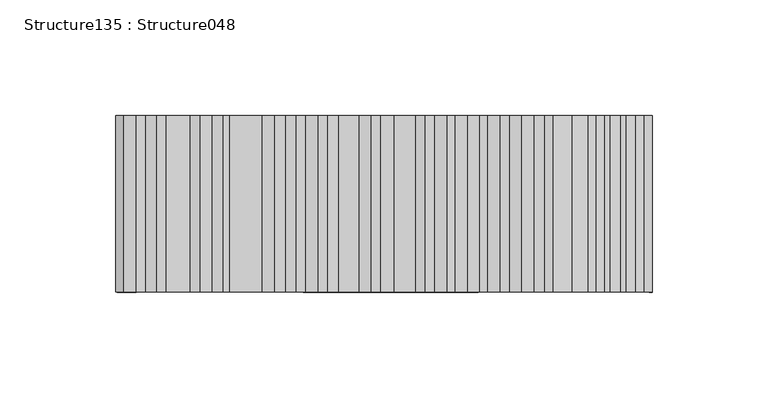
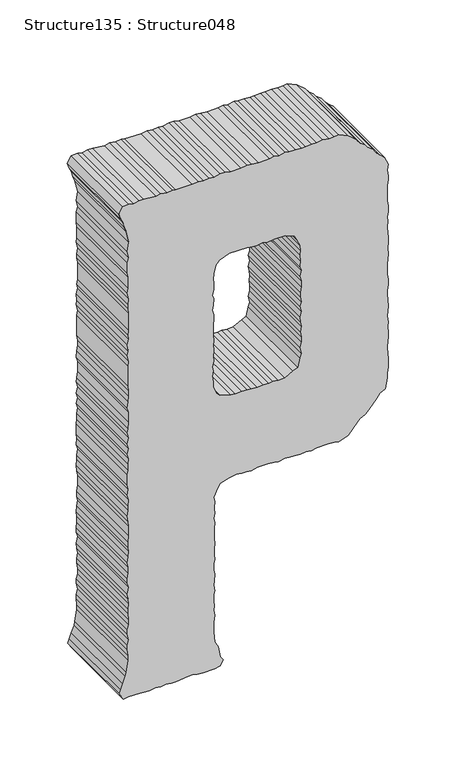
"""IFC4 building model written with IfcOpenShell, lengths in millimetres: proxy geometry, Structure135 : Structure048."""

from ifc_helpers import new_model, si_unit, frame, origin, place, context, project, spatial, polyline, outline, extrude, source, transform, mapped, element, save


def structure135_structure048_a458fe5a(model_context):
    return source(origin(), model_context, "Body", "SweptSolid", [
        extrude(outline(polyline([(3996.390138, -43296.1725089), (3996.390138, -43304.9753692), (3997.5486624, -43309.6560005), (3997.5486624, -43313.755765), (3996.390138, -43319.038123), (3996.9645864, -43323.1394921), (3996.390138, -43327.8185188), (3996.9645864, -43332.5216145), (3996.390138, -43337.7815081), (3996.390138, -43351.8426573), (3996.9645864, -43354.7855019), (3996.390138, -43359.4645286), (3997.5486624, -43364.7244222), (3996.390138, -43368.8482557), (3997.5486624, -43379.3889027), (3997.5486624, -43383.4902717), (3996.390138, -43388.1692985), (3997.5486624, -43392.2706675), (3996.9645864, -43397.5530255), (3991.6806238, -43401.0510633), (3986.4046842, -43399.3132767), (3982.8793681, -43397.5530255), (3978.2035506, -43396.370432), (3973.5197101, -43394.6101809), (3962.9774586, -43392.2706675), (3954.7506513, -43393.4516565), (3948.917914, -43392.2706675), (3944.8165449, -43393.4516565), (3935.4328178, -43393.4516565), (3931.3346579, -43392.8499298), (3921.3748778, -43392.8499298), (3917.2735087, -43393.4516565), (3912.0071968, -43392.2706675), (3906.7328618, -43392.8499298), (3903.2059411, -43392.8499298), (3898.5301236, -43392.2706675), (3883.2863809, -43392.2706675), (3879.1769888, -43392.8499298), (3875.0772243, -43392.2706675), (3870.4030114, -43393.4516565), (3864.5446004, -43392.8499298), (3860.4432313, -43393.4516565), (3855.1769193, -43392.2706675), (3851.0595042, -43392.8499298), (3832.8921721, -43392.8499298), (3828.2163546, -43392.2706675), (3823.5341187, -43392.2706675), (3818.8310229, -43392.8499298), (3812.9726119, -43393.4516565), (3808.8888934, -43392.2706675), (3800.0876378, -43392.2706675), (3794.2292268, -43392.8499298), (3790.7039107, -43393.4516565), (3786.0280932, -43392.2706675), (3780.1616592, -43393.4516565), (3776.0618947, -43392.2706675), (3771.3860772, -43393.4516565), (3766.684586, -43392.2706675), (3762.0023501, -43392.8499298), (3756.7440611, -43392.8499298), (3752.6170184, -43393.4516565), (3743.2332913, -43393.4516565), (3739.1592005, -43392.8499298), (3733.8736333, -43393.4516565), (3729.7738688, -43392.2706675), (3723.9154578, -43392.8499298), (3720.4158154, -43392.8499298), (3715.1302482, -43393.4516565), (3709.8559132, -43392.8499298), (3705.7545441, -43392.2706675), (3696.9709391, -43392.2706675), (3691.0868544, -43392.8499298), (3686.4030139, -43392.8499298), (3682.8857208, -43392.2706675), (3678.2018803, -43392.8499298), (3672.9435914, -43393.4516565), (3668.8261762, -43392.8499298), (3662.9854159, -43392.8499298), (3658.3015753, -43393.4516565), (3654.1841602, -43393.4516565), (3650.1004418, -43392.2706675), (3644.2420307, -43393.4516565), (3639.5405396, -43392.8499298), (3635.4407751, -43392.2706675), (3630.7392839, -43392.8499298), (3626.6571701, -43392.8499298), (3620.7971545, -43392.2706675), (3616.0972679, -43392.2706675), (3612.0135494, -43393.4516565), (3607.8961343, -43393.4516565), (3602.6298224, -43392.2706675), (3597.9540049, -43393.4516565), (3593.8285667, -43393.4516565), (3588.5702778, -43392.8499298), (3584.4689087, -43392.8499298), (3573.9266571, -43394.6101809), (3570.4109687, -43395.2119076), (3564.54293, -43397.5530255), (3559.8671125, -43399.3132767), (3556.3417965, -43400.4718011), (3550.4833855, -43396.9512989), (3551.0658569, -43392.8499298), (3551.0658569, -43382.8885451), (3550.4833855, -43379.3889027), (3550.4833855, -43374.6874115), (3551.0658569, -43369.4275179), (3550.4833855, -43364.7244222), (3551.0658569, -43360.6246577), (3550.4833855, -43355.9440264), (3550.4833855, -43351.8426573), (3551.6675836, -43341.3020103), (3551.6675836, -43337.7815081), (3551.0658569, -43333.680139), (3550.4833855, -43328.4202455), (3550.4833855, -43318.4363963), (3551.6675836, -43313.755765), (3556.3417965, -43311.4162516), (3559.8671125, -43313.755765), (3569.2524442, -43315.5176207), (3575.0851816, -43318.4363963), (3584.4689087, -43319.6173852), (3593.2541183, -43319.6173852), (3599.1125293, -43318.4363963), (3603.7963698, -43319.6173852), (3607.3393366, -43319.038123), (3613.1720739, -43319.6173852), (3617.8559144, -43319.6173852), (3621.3732075, -43318.4363963), (3626.6571701, -43319.6173852), (3630.7392839, -43319.038123), (3636.0408972, -43318.4363963), (3640.7167147, -43319.6173852), (3645.9830266, -43319.6173852), (3649.5003197, -43318.4363963), (3654.7842823, -43319.038123), (3659.4584952, -43319.038123), (3664.1423357, -43318.4363963), (3668.8261762, -43319.038123), (3677.6274319, -43319.038123), (3683.4858429, -43318.4363963), (3687.587212, -43319.6173852), (3691.6869765, -43318.4363963), (3696.3884676, -43319.038123), (3702.229228, -43318.4363963), (3706.3289925, -43319.6173852), (3713.9556777, -43316.0968829), (3716.8985223, -43313.755765), (3719.2316172, -43306.1563581), (3720.4158154, -43300.273878), (3719.8140887, -43295.5932467), (3719.8140887, -43291.4918776), (3719.2316172, -43287.3921131), (3720.4158154, -43282.1097551), (3720.4158154, -43273.3293593), (3719.8140887, -43267.4677391), (3719.2316172, -43263.9472368), (3720.4158154, -43258.6873433), (3719.8140887, -43254.5859742), (3719.8140887, -43248.7259586), (3719.2316172, -43245.2038517), (3719.8140887, -43240.5232204), (3719.2316172, -43235.8217292), (3720.4158154, -43231.1410979), (3720.4158154, -43221.1797132), (3719.8140887, -43215.9198197), (3719.2316172, -43212.3993174), (3722.1568112, -43204.1981838), (3726.8566978, -43200.0968147), (3733.8736333, -43194.2351945), (3736.2163558, -43189.5561678), (3739.1592005, -43186.6133232), (3747.3587295, -43179.570714), (3750.8583719, -43177.2312007), (3753.2171405, -43172.5505694), (3762.5848215, -43170.7903182), (3767.2590344, -43170.7903182), (3771.9605256, -43169.6317938), (3780.1616592, -43169.6317938), (3784.8438951, -43170.211056), (3790.1294623, -43170.7903182), (3795.4037973, -43170.211056), (3799.5051664, -43169.6317938), (3804.1890069, -43169.6317938), (3808.8888934, -43170.211056), (3812.9726119, -43169.6317938), (3818.8310229, -43170.7903182), (3822.348316, -43170.211056), (3827.6162325, -43169.6317938), (3838.1761347, -43170.7903182), (3841.6741725, -43170.7903182), (3846.3772683, -43169.6317938), (3851.6612309, -43169.6317938), (3856.3161885, -43170.7903182), (3865.7015202, -43170.7903182), (3869.8189354, -43170.211056), (3874.5043805, -43169.6317938), (3880.3627915, -43170.211056), (3885.0626781, -43169.6317938), (3889.7208449, -43169.6317938), (3893.822214, -43170.211056), (3899.7046941, -43170.7903182), (3904.3901392, -43170.211056), (3908.46423, -43170.7903182), (3912.5896682, -43169.6317938), (3918.4480792, -43169.6317938), (3923.1319197, -43170.7903182), (3936.6186205, -43170.7903182), (3941.8753048, -43169.6317938), (3945.4182716, -43169.6317938), (3950.6765605, -43170.7903182), (3955.9348494, -43169.6317938), (3963.5615346, -43173.1298316), (3966.5043792, -43176.6519384), (3970.5768654, -43180.7517029), (3974.1214368, -43183.0928209), (3977.6194746, -43187.7718476), (3980.5623192, -43190.1129656), (3983.4794902, -43193.6559323), (3987.5792547, -43197.1555747), (3994.0233463, -43204.1981838), (3997.5486624, -43212.3993174), (3996.9645864, -43215.9198197), (3996.9645864, -43220.600451), (3997.5486624, -43225.8603445), (3996.9645864, -43231.1410979), (3996.9645864, -43235.242467), (3996.390138, -43240.5232204), (3996.390138, -43244.0228628), (3996.9645864, -43249.3052208), (3996.9645864, -43254.5859742), (3997.5486624, -43258.0856166), (3996.390138, -43263.3679746), (3997.5486624, -43267.4677391), (3996.390138, -43271.5691082), (3996.390138, -43280.9512307), (3996.9645864, -43286.8128509), (3997.5486624, -43290.9126154), (3996.390138, -43296.1725089)]), holes=[polyline([(3797.1463977, -43314.3350272), (3799.5051664, -43316.6986096), (3805.9476534, -43319.6173852), (3810.6298893, -43319.6173852), (3816.4883003, -43320.1966474), (3821.1737455, -43319.6173852), (3824.7167122, -43320.1966474), (3829.9733965, -43319.038123), (3834.0474873, -43319.6173852), (3839.3587282, -43319.038123), (3844.6154125, -43319.6173852), (3848.1166595, -43319.038123), (3853.4198774, -43319.6173852), (3862.8036045, -43319.6173852), (3867.4601667, -43319.038123), (3871.5599312, -43319.038123), (3876.263027, -43320.1966474), (3880.3627915, -43319.6173852), (3886.2051565, -43319.038123), (3889.7208449, -43320.1966474), (3894.4030808, -43319.038123), (3899.7046941, -43319.038123), (3904.3901392, -43319.6173852), (3909.0627475, -43319.038123), (3916.0909152, -43317.2778718), (3919.6066036, -43314.3350272), (3922.5494483, -43305.5546314), (3922.5494483, -43290.9126154), (3921.9733953, -43286.2111242), (3921.3748778, -43282.7114818), (3922.5494483, -43277.4291238), (3921.3748778, -43273.3293593), (3921.9733953, -43267.4677391), (3921.9733953, -43258.0856166), (3919.0321552, -43250.4637452), (3915.5068392, -43248.7259586), (3909.0627475, -43245.8055784), (3904.3901392, -43245.2038517), (3900.2887701, -43245.8055784), (3895.0048075, -43245.2038517), (3889.7208449, -43245.8055784), (3886.2051565, -43244.6245895), (3880.9452629, -43245.8055784), (3876.263027, -43244.6245895), (3870.9790644, -43244.6245895), (3866.3032469, -43245.2038517), (3862.2018778, -43245.2038517), (3857.5019912, -43244.6245895), (3854.0007442, -43245.8055784), (3848.7167816, -43244.6245895), (3844.0345457, -43245.8055784), (3839.3587282, -43245.2038517), (3835.2332901, -43244.6245895), (3830.5574726, -43245.2038517), (3825.849563, -43244.6245895), (3821.1737455, -43244.6245895), (3816.4883003, -43245.8055784), (3810.6298893, -43244.6245895), (3807.1045732, -43245.8055784), (3798.9050443, -43247.5433651), (3797.1463977, -43251.6447342), (3793.6451507, -43258.6873433), (3793.0723069, -43263.9472368), (3793.6451507, -43268.648728), (3793.0723069, -43272.1708349), (3793.6451507, -43276.8498616), (3793.0723069, -43282.1097551), (3793.6451507, -43287.3921131), (3793.6451507, -43290.9126154), (3794.2292268, -43295.5932467), (3793.6451507, -43300.8756047), (3794.2292268, -43304.9753692), (3797.1463977, -43314.3350272)])]), frame((0.0, 247945.1599557, 0.0), z_axis=(0.0, 1.0, 0.0), x_axis=(0.0, 0.0, 1.0)), (0.0, 0.0, 1.0), 76.2),
    ])


if __name__ == "__main__":
    model = new_model("IFC4")
    model_context = context("Model", 3, world=origin())
    ifc_project = project(units=[si_unit("LENGTHUNIT", "METRE", prefix="MILLI")], contexts=[model_context])
    site = spatial("IfcSite", under=ifc_project)
    building = spatial("IfcBuilding", under=site)
    placement = place(None, origin())
    structure135_structure048_shape = structure135_structure048_a458fe5a(model_context)
    element("IfcBuildingElementProxy", 1, Name="Structure135 : Structure048", ObjectType="Structure135 : Structure048", at=placement, inside=building, context=model_context, shape_type="MappedRepresentation", body=[
        mapped(structure135_structure048_shape, transform((0.0, 0.0, 0.0), x_axis=(1.0, 0.0, 0.0), y_axis=(0.0, 1.0, 0.0), z_axis=(0.0, 0.0, 1.0))),
    ])
    save(model, "model.ifc")

# Revit data of these elements
# Type "Structure135 : Structure048"
#   NameOverride = "Structure048"
# Element 1 (IfcBuildingElementProxy, "Structure135 : Structure048")
#   Materials on its faces: "BRUSHED ALUM. LETTERING"
# Materials
#   "BRUSHED ALUM. LETTERING": class "Unassigned", colour RGB 169 181 186, transparency 0, Cost = 0
